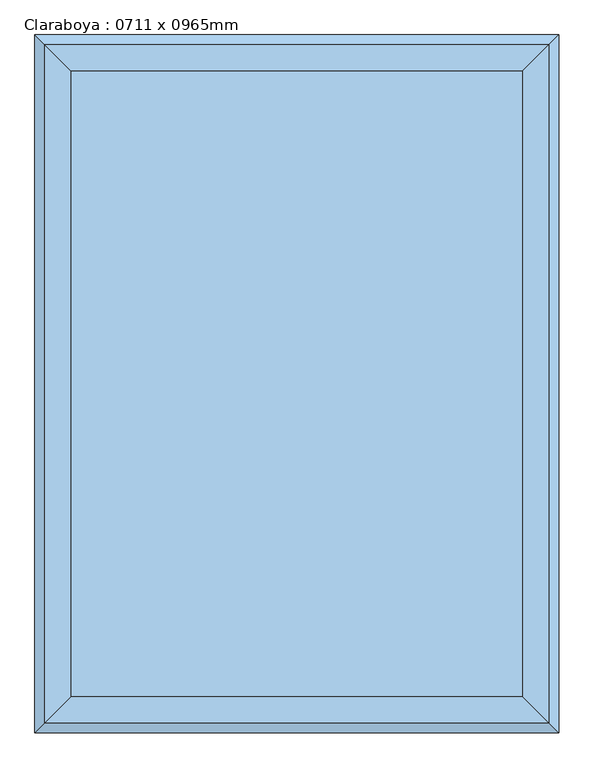
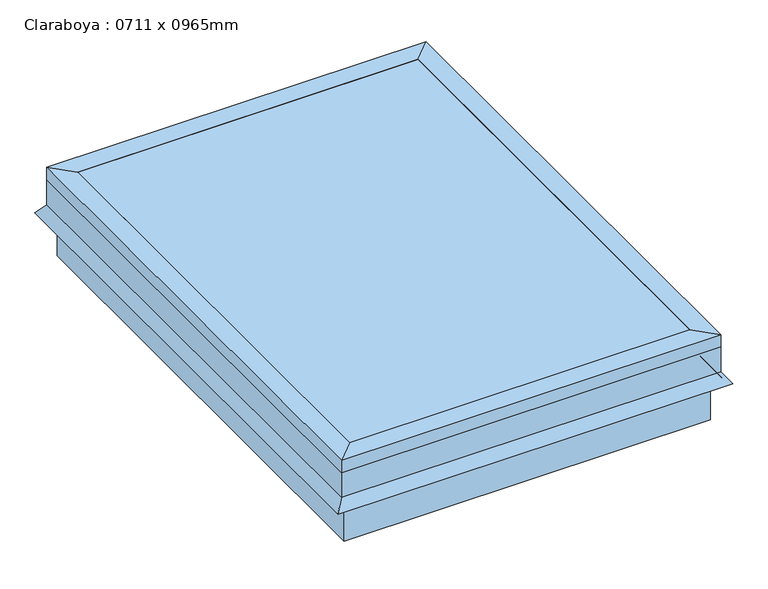
"""IFC4 building model written with IfcOpenShell, lengths in millimetres: window geometry, Claraboya : 0711 x 0965mm."""

from ifc_helpers import new_model, si_unit, frame, origin, place, context, project, spatial, polyline, outline, extrude, faceted_brep, source, transform, mapped, element, save


def claraboya_0711_x_0965mm_17ef4467(model_context):
    return source(origin(), model_context, "Body", "SolidModel", [
        faceted_brep([(254.440073, -370.1040988, 4001.2), (254.440073, 544.0959012, 4001.2), (279.840073, 569.4959012, 4001.2), (279.840073, -395.5040988, 4001.2), (254.440073, -370.1040988, 4026.6), (254.440073, 544.0959012, 4026.6), (292.540073, -408.2040988, 4026.6), (292.540073, 582.1959012, 4026.6), (292.540073, -408.2040988, 4001.2), (292.540073, 582.1959012, 4001.2), (292.540073, -408.2040988, 3950.4), (292.540073, 582.1959012, 3950.4), (307.1089145, -422.7729403, 3929.5935381), (307.1089145, 596.7647427, 3929.5935381), (301.907299, -417.5713248, 3925.9513277), (301.907299, 591.5631272, 3925.9513277), (286.190073, -401.8540988, 3948.3978527), (286.190073, 575.8459012, 3948.3978527), (286.190073, -401.8540988, 4001.2), (286.190073, 575.8459012, 4001.2), (-405.759927, 544.0959012, 4001.2), (-431.159927, 569.4959012, 4001.2), (-405.759927, 544.0959012, 4026.6), (-443.859927, 582.1959012, 4026.6), (-443.859927, 582.1959012, 4001.2), (-443.859927, 582.1959012, 3950.4), (-458.4287685, 596.7647427, 3929.5935381), (-453.227153, 591.5631272, 3925.9513277), (-437.509927, 575.8459012, 3948.3978527), (-437.509927, 575.8459012, 4001.2), (-405.759927, -370.1040988, 4001.2), (-431.159927, -395.5040988, 4001.2), (-405.759927, -370.1040988, 4026.6), (-443.859927, -408.2040988, 4026.6), (-443.859927, -408.2040988, 4001.2), (-443.859927, -408.2040988, 3950.4), (-458.4287685, -422.7729403, 3929.5935381), (-453.227153, -417.5713248, 3925.9513277), (-437.509927, -401.8540988, 3948.3978527), (-437.509927, -401.8540988, 4001.2)], [[[0, 1, 2, 3]], [[4, 5, 1, 0]], [[6, 7, 5, 4]], [[8, 9, 7, 6]], [[10, 11, 9, 8]], [[12, 13, 11, 10]], [[14, 15, 13, 12]], [[16, 17, 15, 14]], [[18, 19, 17, 16]], [[3, 2, 19, 18]], [[1, 20, 21, 2]], [[5, 22, 20, 1]], [[7, 23, 22, 5]], [[9, 24, 23, 7]], [[11, 25, 24, 9]], [[13, 26, 25, 11]], [[15, 27, 26, 13]], [[17, 28, 27, 15]], [[19, 29, 28, 17]], [[2, 21, 29, 19]], [[20, 30, 31, 21]], [[22, 32, 30, 20]], [[23, 33, 32, 22]], [[24, 34, 33, 23]], [[25, 35, 34, 24]], [[26, 36, 35, 25]], [[27, 37, 36, 26]], [[28, 38, 37, 27]], [[29, 39, 38, 28]], [[21, 31, 39, 29]], [[30, 0, 3, 31]], [[32, 4, 0, 30]], [[33, 6, 4, 32]], [[34, 8, 6, 33]], [[35, 10, 8, 34]], [[36, 12, 10, 35]], [[37, 14, 12, 36]], [[38, 16, 14, 37]], [[39, 18, 16, 38]], [[31, 3, 18, 39]]]),
        faceted_brep([(279.840073, 569.4959012, 4001.2), (279.840073, -395.5040988, 4001.2), (279.840073, -395.5040988, 3848.8), (279.840073, 569.4959012, 3848.8), (254.440073, 544.0959012, 4001.2), (254.440073, -370.1040988, 4001.2), (254.440073, 544.0959012, 3975.8), (254.440073, -370.1040988, 3975.8), (235.390073, 525.0459012, 3975.8), (235.390073, -351.0540988, 3975.8), (235.390073, 525.0459012, 3848.8), (235.390073, -351.0540988, 3848.8), (-431.159927, -395.5040988, 4001.2), (-431.159927, -395.5040988, 3848.8), (-405.759927, -370.1040988, 4001.2), (-405.759927, -370.1040988, 3975.8), (-386.709927, -351.0540988, 3975.8), (-386.709927, -351.0540988, 3848.8), (-431.159927, 569.4959012, 4001.2), (-431.159927, 569.4959012, 3848.8), (-405.759927, 544.0959012, 4001.2), (-405.759927, 544.0959012, 3975.8), (-386.709927, 525.0459012, 3975.8), (-386.709927, 525.0459012, 3848.8)], [[[0, 1, 2, 3]], [[4, 5, 1, 0]], [[6, 7, 5, 4]], [[8, 9, 7, 6]], [[10, 11, 9, 8]], [[3, 2, 11, 10]], [[1, 12, 13, 2]], [[5, 14, 12, 1]], [[7, 15, 14, 5]], [[9, 16, 15, 7]], [[11, 17, 16, 9]], [[2, 13, 17, 11]], [[12, 18, 19, 13]], [[14, 20, 18, 12]], [[15, 21, 20, 14]], [[16, 22, 21, 15]], [[17, 23, 22, 16]], [[13, 19, 23, 17]], [[18, 0, 3, 19]], [[20, 4, 0, 18]], [[21, 6, 4, 20]], [[22, 8, 6, 21]], [[23, 10, 8, 22]], [[19, 3, 10, 23]]]),
        extrude(outline(polyline([(254.440073, 544.0959012), (254.440073, -370.1040988), (-405.759927, -370.1040988), (-405.759927, 544.0959012), (254.440073, 544.0959012)])), frame((0.0, 0.0, 4020.25), z_axis=(0.0, 0.0, 1.0), x_axis=(1.0, 0.0, 0.0)), (0.0, 0.0, 1.0), 6.35),
    ])


if __name__ == "__main__":
    model = new_model("IFC4")
    model_context = context("Model", 3, world=origin())
    ifc_project = project(units=[si_unit("LENGTHUNIT", "METRE", prefix="MILLI")], contexts=[model_context])
    site = spatial("IfcSite", under=ifc_project)
    building = spatial("IfcBuilding", under=site)
    placement = place(None, origin())
    claraboya_0711_x_0965mm_shape = claraboya_0711_x_0965mm_17ef4467(model_context)
    element("IfcWindow", 1, ObjectType="Claraboya : 0711 x 0965mm", at=placement, inside=building, context=model_context, shape_type="MappedRepresentation", body=[
        mapped(claraboya_0711_x_0965mm_shape, transform((0.0, 0.0, 0.0), x_axis=(1.0, 0.0, 0.0), y_axis=(0.0, 1.0, 0.0), z_axis=(0.0, 0.0, 1.0))),
    ])
    save(model, "model.ifc")

# Revit data of these elements
# Type "Claraboya : 0711 x 0965mm"
#   Type Mark = "17"
#   Construction Type Id = "GSP4R"
#   Analytic Construction = "1/8 en cristalera simple Pilkington"
#   Visual Light Transmittance = 0.9
#   Solar Heat Gain Coefficient = 0.78
#   Heat Transfer Coefficient (U) = 3.6886 W/(m²·K)
#   Height = 0.965 m
#   Width = 0.711 m
#   Define Thermal Properties by = 1
#   Material de hoja = Metal - Bronce, Bruñido ligero
#   Material de hoja de cristal = Vidrio
#   Material de estructura = Metal - Bronce, Bruñido ligero
#   Type Comments = ""
# Element 1 (IfcWindow, "Claraboya : 0711 x 0965mm")
#   Materials on its faces: "Metal - Bronce, Bruñido ligero", "Vidrio"
# Materials
#   "Metal - Bronce, Bruñido ligero": class "Metal", colour RGB 113 80 70, transparency 0
#   "Vidrio": class "Vidrio", colour RGB 0 128 192, transparency 0.75, Description = "Vidrio de cal sodada", Cost = 0
